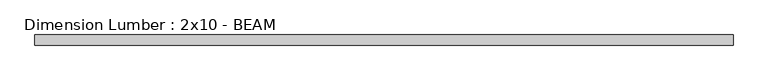
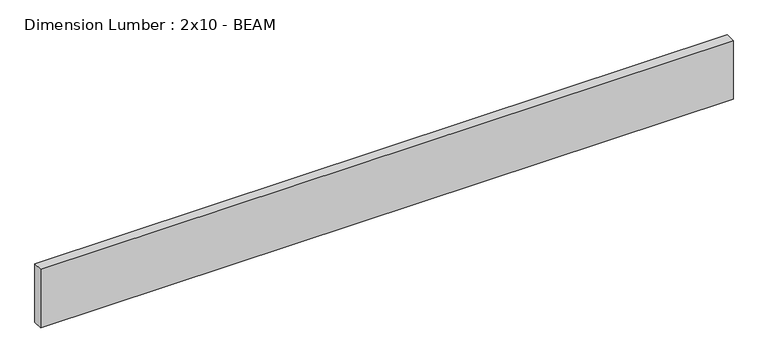
"""IFC4 building model written with IfcOpenShell, lengths in millimetres: beam geometry, Dimension Lumber : 2x10 - BEAM."""

import ifcopenshell
import ifcopenshell.guid

model = None  # the IFC model being written
_history = None  # IfcOwnerHistory: only IFC2X3 demands one
_inside = {}  # id of a spatial element -> (the spatial element, [elements in it])
_under = {}  # id of a project, library or spatial element -> (it, [spatial elements below it])
_declared = {}  # id of a project -> (the project, [libraries it declares])
_typed = {}  # id of a type object -> (the type object, [elements of that type])
_made_of = {}  # id of a material, layer set ... -> (it, [elements and type objects made of it])


def new_model(schema):
    """Start an empty IFC model of exactly this schema.

    Asked for "IFC4X3", IfcOpenShell would pick the latest addendum, in which some entities
    have other attributes; the version numbers below select the first issue.
    IFC2X3 requires an IfcOwnerHistory on every rooted entity: one is made here for all.
    """
    global model, _history
    if schema == "IFC4X3":
        model = ifcopenshell.file(schema_version=(4, 3, 0, 0))
    else:
        model = ifcopenshell.file(schema=schema)
    _inside.clear()
    _under.clear()
    _declared.clear()
    _typed.clear()
    _made_of.clear()
    _history = None
    if model.schema == "IFC2X3":
        org = make("IfcOrganization", Name="unknown")
        user = make(
            "IfcPersonAndOrganization",
            ThePerson=make("IfcPerson", FamilyName="unknown"),
            TheOrganization=org,
        )
        app = make(
            "IfcApplication",
            ApplicationDeveloper=org,
            Version="unknown",
            ApplicationFullName="unknown",
            ApplicationIdentifier="unknown",
        )
        _history = make(
            "IfcOwnerHistory",
            OwningUser=user,
            OwningApplication=app,
            ChangeAction="ADDED",
            CreationDate=0,
        )
    return model


def make(cls, **values):
    """One entity of the class cls with the attributes given. An attribute that is None is left unset."""
    return model.create_entity(
        cls, **{name: value for name, value in values.items() if value is not None}
    )


def rooted(cls, **values):
    """An entity with a GlobalId (a new one), such as an element, a storey or a relation."""
    return make(cls, GlobalId=ifcopenshell.guid.new(), OwnerHistory=_history, **values)


def si_unit(unit_type, name, prefix=None):
    """IfcSIUnit, for example si_unit("LENGTHUNIT", "METRE", prefix="MILLI")."""
    return make("IfcSIUnit", UnitType=unit_type, Prefix=prefix, Name=name)


def assignment(units):
    """IfcUnitAssignment: the units of a project."""
    return None if units is None else make("IfcUnitAssignment", Units=units)


def point(xyz):
    """IfcCartesianPoint."""
    return None if xyz is None else make("IfcCartesianPoint", Coordinates=xyz)


def direction(xyz):
    """IfcDirection."""
    return None if xyz is None else make("IfcDirection", DirectionRatios=xyz)


def frame(location, z_axis=None, x_axis=None):
    """IfcAxis2Placement3D, a coordinate frame: its origin and axes. An axis left out is left unset."""
    return make(
        "IfcAxis2Placement3D",
        Location=point(location),
        Axis=direction(z_axis),
        RefDirection=direction(x_axis),
    )


def origin():
    """The frame at (0, 0, 0) with its axes left unset."""
    return frame((0.0, 0.0, 0.0))


def place(relative_to, where):
    """IfcLocalPlacement: puts the frame where relative to a parent placement (None: the world)."""
    return make(
        "IfcLocalPlacement", PlacementRelTo=relative_to, RelativePlacement=where
    )


def context(
    kind, dimensions, precision=None, world=None, true_north=None, identifier=None
):
    """IfcGeometricRepresentationContext, for example the 3D "Model" context."""
    return make(
        "IfcGeometricRepresentationContext",
        ContextIdentifier=identifier,
        ContextType=kind,
        CoordinateSpaceDimension=dimensions,
        Precision=precision,
        WorldCoordinateSystem=world,
        TrueNorth=true_north,
    )


def project(units=None, contexts=None):
    """IfcProject with its units and contexts."""
    return rooted(
        "IfcProject",
        Name="project",
        RepresentationContexts=contexts,
        UnitsInContext=assignment(units),
    )


def spatial(cls, under=None, at=None, **own):
    """A site, building, storey or space (cls), placed at a placement, below another one or the project."""
    s = rooted(cls, ObjectPlacement=at, **own)
    if under is not None:
        _under.setdefault(under.id(), (under, []))[1].append(s)
    return s


def polyline(points):
    """IfcPolyline through the points."""
    return make("IfcPolyline", Points=[point(p) for p in points])


def outline(outer, holes=None, kind="AREA"):
    """IfcArbitraryClosedProfileDef: a profile drawn as a closed curve; with holes, ...WithVoids."""
    if holes is None:
        return make("IfcArbitraryClosedProfileDef", ProfileType=kind, OuterCurve=outer)
    return make(
        "IfcArbitraryProfileDefWithVoids",
        ProfileType=kind,
        OuterCurve=outer,
        InnerCurves=holes,
    )


def extrude(swept, where, along, depth):
    """IfcExtrudedAreaSolid: the profile swept, set in the frame where, extruded along a direction by depth."""
    return make(
        "IfcExtrudedAreaSolid",
        SweptArea=swept,
        Position=where,
        ExtrudedDirection=direction(along),
        Depth=depth,
    )


def shape(context_of_items, identifier, shape_type, items):
    """IfcShapeRepresentation: the items that make up one representation, for example the "Body"."""
    return make(
        "IfcShapeRepresentation",
        ContextOfItems=context_of_items,
        RepresentationIdentifier=identifier,
        RepresentationType=shape_type,
        Items=items,
    )


def source(mapping_origin, context_of_items, identifier, shape_type, items):
    """IfcRepresentationMap: a shape defined once, which mapped items show again and again."""
    return make(
        "IfcRepresentationMap",
        MappingOrigin=mapping_origin,
        MappedRepresentation=shape(context_of_items, identifier, shape_type, items),
    )


def transform(
    local_origin,
    x_axis=None,
    y_axis=None,
    z_axis=None,
    scale=None,
    scale2=None,
    scale3=None,
    uniform=True,
):
    """IfcCartesianTransformationOperator3D, or its non-uniform kind. x_axis, y_axis, z_axis: its Axis1, 2, 3."""
    if uniform:
        return make(
            "IfcCartesianTransformationOperator3D",
            Axis1=direction(x_axis),
            Axis2=direction(y_axis),
            LocalOrigin=point(local_origin),
            Scale=scale,
            Axis3=direction(z_axis),
        )
    return make(
        "IfcCartesianTransformationOperator3DnonUniform",
        Axis1=direction(x_axis),
        Axis2=direction(y_axis),
        LocalOrigin=point(local_origin),
        Scale=scale,
        Axis3=direction(z_axis),
        Scale2=scale2,
        Scale3=scale3,
    )


def mapped(mapping_source, mapping_target):
    """IfcMappedItem: shows the shape of a source again, moved by a transform."""
    return make(
        "IfcMappedItem", MappingSource=mapping_source, MappingTarget=mapping_target
    )


def made_of(thing, what):
    """Note that an element or type object is made of a material, layer set ...; save() writes the relation."""
    if what is not None:
        _made_of.setdefault(what.id(), (what, []))[1].append(thing)
    return thing


def element(
    cls,
    number,
    at=None,
    inside=None,
    cuts=None,
    type_object=None,
    material=None,
    context=None,
    identifier="Body",
    shape_type=None,
    held_by="IfcProductDefinitionShape",
    body=None,
    shapes=None,
    **own,
):
    """One element of the class cls, such as IfcWall. Its Tag is "e" and its number.

    at: its placement. inside: the storey or other place that contains it. cuts: it is an
    opening in that element (IfcRelVoidsElement). A single representation is given by context,
    identifier, shape_type and body (its items); several are given by shapes. held_by: the class
    of the entity that holds the representations. save() writes the other relations.
    """
    e = rooted(cls, Tag="e%d" % number, ObjectPlacement=at, **own)
    if body is not None:
        shapes = [shape(context, identifier, shape_type, body)]
    if shapes is not None:
        e.Representation = make(held_by, Representations=shapes)
    if inside is not None:
        _inside.setdefault(inside.id(), (inside, []))[1].append(e)
    if cuts is not None:
        rooted(
            "IfcRelVoidsElement", RelatingBuildingElement=cuts, RelatedOpeningElement=e
        )
    if type_object is not None:
        _typed.setdefault(type_object.id(), (type_object, []))[1].append(e)
    return made_of(e, material)


def aggregate(whole, parts):
    """IfcRelAggregates: a whole, such as a stair, and the parts it consists of."""
    return rooted("IfcRelAggregates", RelatingObject=whole, RelatedObjects=parts)


def save(model, path):
    """Write the relations noted so far, then the file.

    IfcRelAggregates (storeys below a building ...), IfcRelContainedInSpatialStructure (elements
    in a storey), IfcRelDefinesByType, IfcRelAssociatesMaterial and IfcRelDeclares: one each for
    every whole, place, type object, material and project.
    """
    for whole, parts in _under.values():
        aggregate(whole, parts)
    for where, things in _inside.values():
        rooted(
            "IfcRelContainedInSpatialStructure",
            RelatedElements=things,
            RelatingStructure=where,
        )
    for kind, things in _typed.values():
        rooted("IfcRelDefinesByType", RelatedObjects=things, RelatingType=kind)
    for what, things in _made_of.values():
        rooted("IfcRelAssociatesMaterial", RelatedObjects=things, RelatingMaterial=what)
    for by, libraries in _declared.values():
        rooted("IfcRelDeclares", RelatingContext=by, RelatedDefinitions=libraries)
    model.write(path)


def dimension_lumber_2x10_beam_b235e4ad(model_context):
    return source(origin(), model_context, "Body", "SweptSolid", [
        extrude(outline(polyline([(1314.45, 19.05), (1314.45, -19.05), (-1314.45, -19.05), (-1314.45, 19.05), (1314.45, 19.05)])), frame((0.0, 0.0, -117.475), z_axis=(0.0, 0.0, 1.0), x_axis=(1.0, 0.0, 0.0)), (0.0, 0.0, 1.0), 234.95),
    ])


if __name__ == "__main__":
    model = new_model("IFC4")
    model_context = context("Model", 3, world=origin())
    ifc_project = project(units=[si_unit("LENGTHUNIT", "METRE", prefix="MILLI")], contexts=[model_context])
    site = spatial("IfcSite", under=ifc_project)
    building = spatial("IfcBuilding", under=site)
    placement = place(None, origin())
    dimension_lumber_2x10_beam_shape = dimension_lumber_2x10_beam_b235e4ad(model_context)
    element("IfcBeam", 1, ObjectType="Dimension Lumber : 2x10 - BEAM", at=placement, inside=building, context=model_context, shape_type="MappedRepresentation", body=[
        mapped(dimension_lumber_2x10_beam_shape, transform((0.0, 0.0, 0.0), x_axis=(1.0, 0.0, 0.0), y_axis=(0.0, 1.0, 0.0), z_axis=(0.0, 0.0, 1.0))),
    ])
    save(model, "model.ifc")

# Revit data of these elements
# Type "Dimension Lumber : 2x10 - BEAM"
#   Assembly Code = "B10"
#   A = 0.0755556 SF
#   Length [instance default] = 5' - 0"
#   b = 0' - 1 1/2"
#   d = 0' - 9 1/4"
#   Structural Material = (3) SISTERED 2X10s AT BEAM
# Element 1 (IfcBeam, "Dimension Lumber : 2x10 - BEAM")
#   Materials on its faces: "(3) SISTERED 2X10s AT BEAM"
# Materials
#   "(3) SISTERED 2X10s AT BEAM": class "Wood", colour RGB 234 198 147, transparency 0, Description = "Pinus Echinata", Cost = 0
